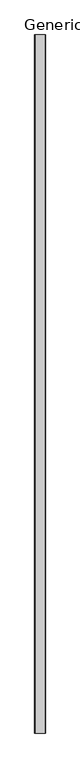
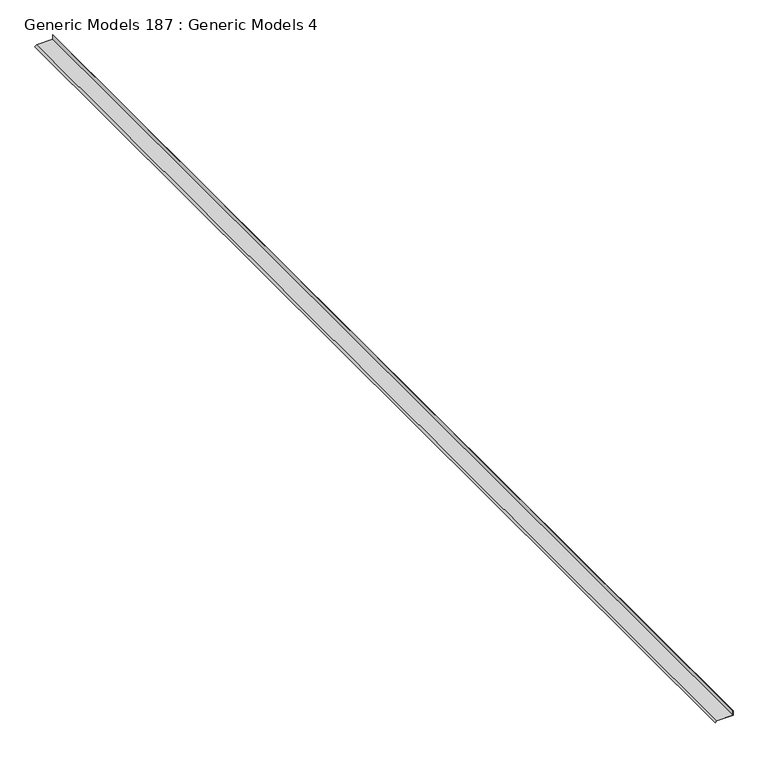
"""IFC4 building model written with IfcOpenShell, lengths in millimetres: proxy geometry, Generic Models 187 : Generic Models 4."""

from ifc_helpers import new_model, si_unit, frame, origin, place, context, project, spatial, polyline, outline, extrude, source, transform, mapped, element, save


def generic_models_187_generic_models_4_ea36ebd6(model_context):
    return source(origin(), model_context, "Body", "SweptSolid", [
        extrude(outline(polyline([(126767.17725, -5226.8751963), (126799.721, -5226.8751963), (126799.721, -5227.6689463), (126767.971, -5227.6689463), (126767.971, -5336.1156256), (126756.7456798, -5347.3409458), (126756.1844138, -5346.7796798), (126767.17725, -5335.7868436), (126767.17725, -5226.8751963)])), frame((0.0, -464.1230338, 0.0), z_axis=(0.0, 1.0, 0.0), x_axis=(0.0, 0.0, 1.0)), (0.0, 0.0, 1.0), 7886.7),
    ])


if __name__ == "__main__":
    model = new_model("IFC4")
    model_context = context("Model", 3, world=origin())
    ifc_project = project(units=[si_unit("LENGTHUNIT", "METRE", prefix="MILLI")], contexts=[model_context])
    site = spatial("IfcSite", under=ifc_project)
    building = spatial("IfcBuilding", under=site)
    placement = place(None, origin())
    generic_models_187_generic_models_4_shape = generic_models_187_generic_models_4_ea36ebd6(model_context)
    element("IfcBuildingElementProxy", 1, Name="Generic Models 187 : Generic Models 4", ObjectType="Generic Models 187 : Generic Models 4", at=placement, inside=building, context=model_context, shape_type="MappedRepresentation", body=[
        mapped(generic_models_187_generic_models_4_shape, transform((0.0, 0.0, 0.0), x_axis=(1.0, 0.0, 0.0), y_axis=(0.0, 1.0, 0.0), z_axis=(0.0, 0.0, 1.0))),
    ])
    save(model, "model.ifc")

# Revit data of these elements
# Element 1 (IfcBuildingElementProxy, "Generic Models 187 : Generic Models 4")
#   Materials on its faces: "_12 GAUGE S.S. FLASHING WITH END DAMS"
# Materials
#   "_12 GAUGE S.S. FLASHING WITH END DAMS": class "Generic", colour RGB 67 154 161, transparency 0, Cost = 0
